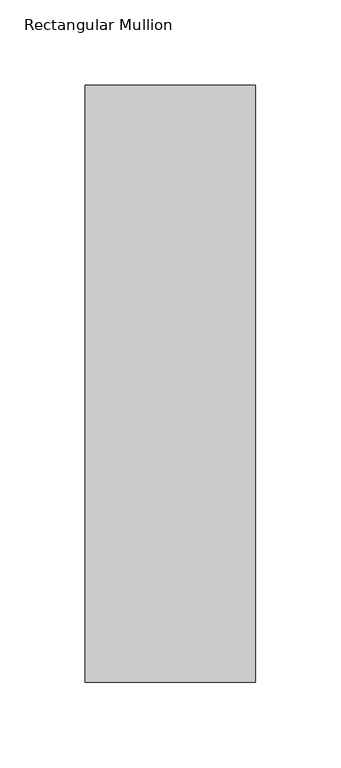
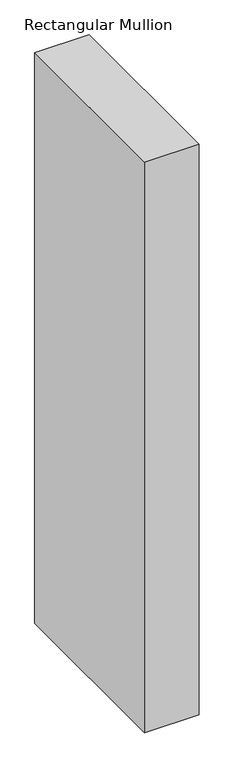
"""IFC4 building model written with IfcOpenShell, lengths in millimetres: member geometry, Rectangular Mullion : WWm-100x350-100mmOffset."""

import ifcopenshell
import ifcopenshell.guid

model = None  # the IFC model being written
_history = None  # IfcOwnerHistory: only IFC2X3 demands one
_inside = {}  # id of a spatial element -> (the spatial element, [elements in it])
_under = {}  # id of a project, library or spatial element -> (it, [spatial elements below it])
_declared = {}  # id of a project -> (the project, [libraries it declares])
_typed = {}  # id of a type object -> (the type object, [elements of that type])
_made_of = {}  # id of a material, layer set ... -> (it, [elements and type objects made of it])


def new_model(schema):
    """Start an empty IFC model of exactly this schema.

    Asked for "IFC4X3", IfcOpenShell would pick the latest addendum, in which some entities
    have other attributes; the version numbers below select the first issue.
    IFC2X3 requires an IfcOwnerHistory on every rooted entity: one is made here for all.
    """
    global model, _history
    if schema == "IFC4X3":
        model = ifcopenshell.file(schema_version=(4, 3, 0, 0))
    else:
        model = ifcopenshell.file(schema=schema)
    _inside.clear()
    _under.clear()
    _declared.clear()
    _typed.clear()
    _made_of.clear()
    _history = None
    if model.schema == "IFC2X3":
        org = make("IfcOrganization", Name="unknown")
        user = make(
            "IfcPersonAndOrganization",
            ThePerson=make("IfcPerson", FamilyName="unknown"),
            TheOrganization=org,
        )
        app = make(
            "IfcApplication",
            ApplicationDeveloper=org,
            Version="unknown",
            ApplicationFullName="unknown",
            ApplicationIdentifier="unknown",
        )
        _history = make(
            "IfcOwnerHistory",
            OwningUser=user,
            OwningApplication=app,
            ChangeAction="ADDED",
            CreationDate=0,
        )
    return model


def make(cls, **values):
    """One entity of the class cls with the attributes given. An attribute that is None is left unset."""
    return model.create_entity(
        cls, **{name: value for name, value in values.items() if value is not None}
    )


def rooted(cls, **values):
    """An entity with a GlobalId (a new one), such as an element, a storey or a relation."""
    return make(cls, GlobalId=ifcopenshell.guid.new(), OwnerHistory=_history, **values)


def si_unit(unit_type, name, prefix=None):
    """IfcSIUnit, for example si_unit("LENGTHUNIT", "METRE", prefix="MILLI")."""
    return make("IfcSIUnit", UnitType=unit_type, Prefix=prefix, Name=name)


def assignment(units):
    """IfcUnitAssignment: the units of a project."""
    return None if units is None else make("IfcUnitAssignment", Units=units)


def point(xyz):
    """IfcCartesianPoint."""
    return None if xyz is None else make("IfcCartesianPoint", Coordinates=xyz)


def direction(xyz):
    """IfcDirection."""
    return None if xyz is None else make("IfcDirection", DirectionRatios=xyz)


def frame(location, z_axis=None, x_axis=None):
    """IfcAxis2Placement3D, a coordinate frame: its origin and axes. An axis left out is left unset."""
    return make(
        "IfcAxis2Placement3D",
        Location=point(location),
        Axis=direction(z_axis),
        RefDirection=direction(x_axis),
    )


def origin():
    """The frame at (0, 0, 0) with its axes left unset."""
    return frame((0.0, 0.0, 0.0))


def place(relative_to, where):
    """IfcLocalPlacement: puts the frame where relative to a parent placement (None: the world)."""
    return make(
        "IfcLocalPlacement", PlacementRelTo=relative_to, RelativePlacement=where
    )


def context(
    kind, dimensions, precision=None, world=None, true_north=None, identifier=None
):
    """IfcGeometricRepresentationContext, for example the 3D "Model" context."""
    return make(
        "IfcGeometricRepresentationContext",
        ContextIdentifier=identifier,
        ContextType=kind,
        CoordinateSpaceDimension=dimensions,
        Precision=precision,
        WorldCoordinateSystem=world,
        TrueNorth=true_north,
    )


def project(units=None, contexts=None):
    """IfcProject with its units and contexts."""
    return rooted(
        "IfcProject",
        Name="project",
        RepresentationContexts=contexts,
        UnitsInContext=assignment(units),
    )


def spatial(cls, under=None, at=None, **own):
    """A site, building, storey or space (cls), placed at a placement, below another one or the project."""
    s = rooted(cls, ObjectPlacement=at, **own)
    if under is not None:
        _under.setdefault(under.id(), (under, []))[1].append(s)
    return s


def polyline(points):
    """IfcPolyline through the points."""
    return make("IfcPolyline", Points=[point(p) for p in points])


def outline(outer, holes=None, kind="AREA"):
    """IfcArbitraryClosedProfileDef: a profile drawn as a closed curve; with holes, ...WithVoids."""
    if holes is None:
        return make("IfcArbitraryClosedProfileDef", ProfileType=kind, OuterCurve=outer)
    return make(
        "IfcArbitraryProfileDefWithVoids",
        ProfileType=kind,
        OuterCurve=outer,
        InnerCurves=holes,
    )


def extrude(swept, where, along, depth):
    """IfcExtrudedAreaSolid: the profile swept, set in the frame where, extruded along a direction by depth."""
    return make(
        "IfcExtrudedAreaSolid",
        SweptArea=swept,
        Position=where,
        ExtrudedDirection=direction(along),
        Depth=depth,
    )


def shape(context_of_items, identifier, shape_type, items):
    """IfcShapeRepresentation: the items that make up one representation, for example the "Body"."""
    return make(
        "IfcShapeRepresentation",
        ContextOfItems=context_of_items,
        RepresentationIdentifier=identifier,
        RepresentationType=shape_type,
        Items=items,
    )


def source(mapping_origin, context_of_items, identifier, shape_type, items):
    """IfcRepresentationMap: a shape defined once, which mapped items show again and again."""
    return make(
        "IfcRepresentationMap",
        MappingOrigin=mapping_origin,
        MappedRepresentation=shape(context_of_items, identifier, shape_type, items),
    )


def transform(
    local_origin,
    x_axis=None,
    y_axis=None,
    z_axis=None,
    scale=None,
    scale2=None,
    scale3=None,
    uniform=True,
):
    """IfcCartesianTransformationOperator3D, or its non-uniform kind. x_axis, y_axis, z_axis: its Axis1, 2, 3."""
    if uniform:
        return make(
            "IfcCartesianTransformationOperator3D",
            Axis1=direction(x_axis),
            Axis2=direction(y_axis),
            LocalOrigin=point(local_origin),
            Scale=scale,
            Axis3=direction(z_axis),
        )
    return make(
        "IfcCartesianTransformationOperator3DnonUniform",
        Axis1=direction(x_axis),
        Axis2=direction(y_axis),
        LocalOrigin=point(local_origin),
        Scale=scale,
        Axis3=direction(z_axis),
        Scale2=scale2,
        Scale3=scale3,
    )


def mapped(mapping_source, mapping_target):
    """IfcMappedItem: shows the shape of a source again, moved by a transform."""
    return make(
        "IfcMappedItem", MappingSource=mapping_source, MappingTarget=mapping_target
    )


def made_of(thing, what):
    """Note that an element or type object is made of a material, layer set ...; save() writes the relation."""
    if what is not None:
        _made_of.setdefault(what.id(), (what, []))[1].append(thing)
    return thing


def element(
    cls,
    number,
    at=None,
    inside=None,
    cuts=None,
    type_object=None,
    material=None,
    context=None,
    identifier="Body",
    shape_type=None,
    held_by="IfcProductDefinitionShape",
    body=None,
    shapes=None,
    **own,
):
    """One element of the class cls, such as IfcWall. Its Tag is "e" and its number.

    at: its placement. inside: the storey or other place that contains it. cuts: it is an
    opening in that element (IfcRelVoidsElement). A single representation is given by context,
    identifier, shape_type and body (its items); several are given by shapes. held_by: the class
    of the entity that holds the representations. save() writes the other relations.
    """
    e = rooted(cls, Tag="e%d" % number, ObjectPlacement=at, **own)
    if body is not None:
        shapes = [shape(context, identifier, shape_type, body)]
    if shapes is not None:
        e.Representation = make(held_by, Representations=shapes)
    if inside is not None:
        _inside.setdefault(inside.id(), (inside, []))[1].append(e)
    if cuts is not None:
        rooted(
            "IfcRelVoidsElement", RelatingBuildingElement=cuts, RelatedOpeningElement=e
        )
    if type_object is not None:
        _typed.setdefault(type_object.id(), (type_object, []))[1].append(e)
    return made_of(e, material)


def aggregate(whole, parts):
    """IfcRelAggregates: a whole, such as a stair, and the parts it consists of."""
    return rooted("IfcRelAggregates", RelatingObject=whole, RelatedObjects=parts)


def save(model, path):
    """Write the relations noted so far, then the file.

    IfcRelAggregates (storeys below a building ...), IfcRelContainedInSpatialStructure (elements
    in a storey), IfcRelDefinesByType, IfcRelAssociatesMaterial and IfcRelDeclares: one each for
    every whole, place, type object, material and project.
    """
    for whole, parts in _under.values():
        aggregate(whole, parts)
    for where, things in _inside.values():
        rooted(
            "IfcRelContainedInSpatialStructure",
            RelatedElements=things,
            RelatingStructure=where,
        )
    for kind, things in _typed.values():
        rooted("IfcRelDefinesByType", RelatedObjects=things, RelatingType=kind)
    for what, things in _made_of.values():
        rooted("IfcRelAssociatesMaterial", RelatedObjects=things, RelatingMaterial=what)
    for by, libraries in _declared.values():
        rooted("IfcRelDeclares", RelatingContext=by, RelatedDefinitions=libraries)
    model.write(path)


def rectangular_mullion_f67b7a8e(model_context):
    return source(origin(), model_context, "Body", "SweptSolid", [
        extrude(outline(polyline([(0.0, 175.0), (0.0, -175.0), (-100.0, -175.0), (-100.0, 175.0), (0.0, 175.0)])), frame((0.0, 0.0, -1110.0), z_axis=(0.0, 0.0, 1.0), x_axis=(1.0, 0.0, 0.0)), (0.0, 0.0, 1.0), 1110.0),
    ])


if __name__ == "__main__":
    model = new_model("IFC4")
    model_context = context("Model", 3, world=origin())
    ifc_project = project(units=[si_unit("LENGTHUNIT", "METRE", prefix="MILLI")], contexts=[model_context])
    site = spatial("IfcSite", under=ifc_project)
    building = spatial("IfcBuilding", under=site)
    placement = place(None, origin())
    rectangular_mullion_shape = rectangular_mullion_f67b7a8e(model_context)
    element("IfcMember", 1, ObjectType="Rectangular Mullion : WWm-100x350-100mmOffset", at=placement, inside=building, context=model_context, shape_type="MappedRepresentation", body=[
        mapped(rectangular_mullion_shape, transform((0.0, 0.0, 0.0), x_axis=(1.0, 0.0, 0.0), y_axis=(0.0, 1.0, 0.0), z_axis=(0.0, 0.0, 1.0))),
    ])
    save(model, "model.ifc")

# Revit data of these elements
# Type "Rectangular Mullion : WWm-100x350-100mmOffset"
#   built-in parameter 1007304 = 1.14829 (stored number, unit not read)
#   built-in parameter 1007301 = 0.164042 (stored number, unit not read)
#   built-in parameter 1007300 = 0.164042 (stored number, unit not read)
# Element 1 (IfcMember, "Rectangular Mullion : WWm-100x350-100mmOffset")
#   Materials on its faces: "WW-EC-RGB-Mullion"
# Materials
#   "WW-EC-RGB-Mullion": class "Generic", colour RGB 255 255 255, transparency 0, Comments = "If region requests black mullions, switch asset color to RGB 25-25-25", Description = "Generic Color", Cost = 0
